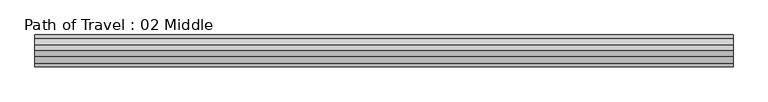
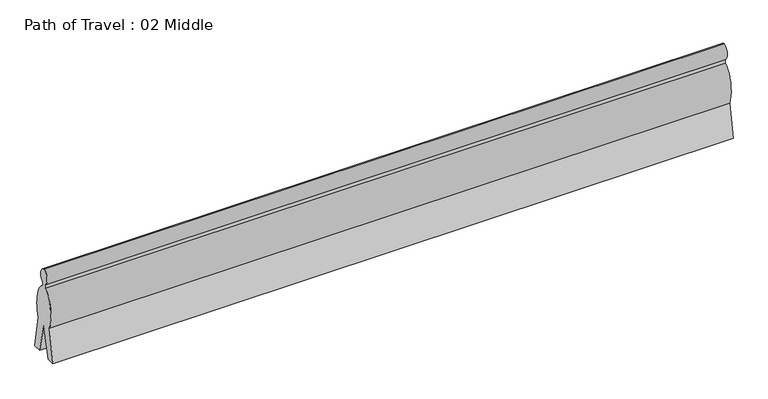
"""IFC4 building model written with IfcOpenShell, lengths in millimetres: proxy geometry, Path of Travel : 02 Middle."""

import ifcopenshell
import ifcopenshell.guid

model = None  # the IFC model being written
_history = None  # IfcOwnerHistory: only IFC2X3 demands one
_inside = {}  # id of a spatial element -> (the spatial element, [elements in it])
_under = {}  # id of a project, library or spatial element -> (it, [spatial elements below it])
_declared = {}  # id of a project -> (the project, [libraries it declares])
_typed = {}  # id of a type object -> (the type object, [elements of that type])
_made_of = {}  # id of a material, layer set ... -> (it, [elements and type objects made of it])


def new_model(schema):
    """Start an empty IFC model of exactly this schema.

    Asked for "IFC4X3", IfcOpenShell would pick the latest addendum, in which some entities
    have other attributes; the version numbers below select the first issue.
    IFC2X3 requires an IfcOwnerHistory on every rooted entity: one is made here for all.
    """
    global model, _history
    if schema == "IFC4X3":
        model = ifcopenshell.file(schema_version=(4, 3, 0, 0))
    else:
        model = ifcopenshell.file(schema=schema)
    _inside.clear()
    _under.clear()
    _declared.clear()
    _typed.clear()
    _made_of.clear()
    _history = None
    if model.schema == "IFC2X3":
        org = make("IfcOrganization", Name="unknown")
        user = make(
            "IfcPersonAndOrganization",
            ThePerson=make("IfcPerson", FamilyName="unknown"),
            TheOrganization=org,
        )
        app = make(
            "IfcApplication",
            ApplicationDeveloper=org,
            Version="unknown",
            ApplicationFullName="unknown",
            ApplicationIdentifier="unknown",
        )
        _history = make(
            "IfcOwnerHistory",
            OwningUser=user,
            OwningApplication=app,
            ChangeAction="ADDED",
            CreationDate=0,
        )
    return model


def make(cls, **values):
    """One entity of the class cls with the attributes given. An attribute that is None is left unset."""
    return model.create_entity(
        cls, **{name: value for name, value in values.items() if value is not None}
    )


def rooted(cls, **values):
    """An entity with a GlobalId (a new one), such as an element, a storey or a relation."""
    return make(cls, GlobalId=ifcopenshell.guid.new(), OwnerHistory=_history, **values)


def si_unit(unit_type, name, prefix=None):
    """IfcSIUnit, for example si_unit("LENGTHUNIT", "METRE", prefix="MILLI")."""
    return make("IfcSIUnit", UnitType=unit_type, Prefix=prefix, Name=name)


def assignment(units):
    """IfcUnitAssignment: the units of a project."""
    return None if units is None else make("IfcUnitAssignment", Units=units)


def point(xyz):
    """IfcCartesianPoint."""
    return None if xyz is None else make("IfcCartesianPoint", Coordinates=xyz)


def direction(xyz):
    """IfcDirection."""
    return None if xyz is None else make("IfcDirection", DirectionRatios=xyz)


def frame(location, z_axis=None, x_axis=None):
    """IfcAxis2Placement3D, a coordinate frame: its origin and axes. An axis left out is left unset."""
    return make(
        "IfcAxis2Placement3D",
        Location=point(location),
        Axis=direction(z_axis),
        RefDirection=direction(x_axis),
    )


def origin():
    """The frame at (0, 0, 0) with its axes left unset."""
    return frame((0.0, 0.0, 0.0))


def place(relative_to, where):
    """IfcLocalPlacement: puts the frame where relative to a parent placement (None: the world)."""
    return make(
        "IfcLocalPlacement", PlacementRelTo=relative_to, RelativePlacement=where
    )


def context(
    kind, dimensions, precision=None, world=None, true_north=None, identifier=None
):
    """IfcGeometricRepresentationContext, for example the 3D "Model" context."""
    return make(
        "IfcGeometricRepresentationContext",
        ContextIdentifier=identifier,
        ContextType=kind,
        CoordinateSpaceDimension=dimensions,
        Precision=precision,
        WorldCoordinateSystem=world,
        TrueNorth=true_north,
    )


def project(units=None, contexts=None):
    """IfcProject with its units and contexts."""
    return rooted(
        "IfcProject",
        Name="project",
        RepresentationContexts=contexts,
        UnitsInContext=assignment(units),
    )


def spatial(cls, under=None, at=None, **own):
    """A site, building, storey or space (cls), placed at a placement, below another one or the project."""
    s = rooted(cls, ObjectPlacement=at, **own)
    if under is not None:
        _under.setdefault(under.id(), (under, []))[1].append(s)
    return s


def ellipse_curve(where, semi_axis1, semi_axis2):
    """IfcEllipse in the frame where."""
    return make(
        "IfcEllipse", Position=where, SemiAxis1=semi_axis1, SemiAxis2=semi_axis2
    )


def trimmed(basis, trim1, trim2, sense, master):
    """IfcTrimmedCurve: the piece of a basis curve between two trims."""
    return make(
        "IfcTrimmedCurve",
        BasisCurve=basis,
        Trim1=trim1,
        Trim2=trim2,
        SenseAgreement=sense,
        MasterRepresentation=master,
    )


def shape(context_of_items, identifier, shape_type, items):
    """IfcShapeRepresentation: the items that make up one representation, for example the "Body"."""
    return make(
        "IfcShapeRepresentation",
        ContextOfItems=context_of_items,
        RepresentationIdentifier=identifier,
        RepresentationType=shape_type,
        Items=items,
    )


def source(mapping_origin, context_of_items, identifier, shape_type, items):
    """IfcRepresentationMap: a shape defined once, which mapped items show again and again."""
    return make(
        "IfcRepresentationMap",
        MappingOrigin=mapping_origin,
        MappedRepresentation=shape(context_of_items, identifier, shape_type, items),
    )


def transform(
    local_origin,
    x_axis=None,
    y_axis=None,
    z_axis=None,
    scale=None,
    scale2=None,
    scale3=None,
    uniform=True,
):
    """IfcCartesianTransformationOperator3D, or its non-uniform kind. x_axis, y_axis, z_axis: its Axis1, 2, 3."""
    if uniform:
        return make(
            "IfcCartesianTransformationOperator3D",
            Axis1=direction(x_axis),
            Axis2=direction(y_axis),
            LocalOrigin=point(local_origin),
            Scale=scale,
            Axis3=direction(z_axis),
        )
    return make(
        "IfcCartesianTransformationOperator3DnonUniform",
        Axis1=direction(x_axis),
        Axis2=direction(y_axis),
        LocalOrigin=point(local_origin),
        Scale=scale,
        Axis3=direction(z_axis),
        Scale2=scale2,
        Scale3=scale3,
    )


def mapped(mapping_source, mapping_target):
    """IfcMappedItem: shows the shape of a source again, moved by a transform."""
    return make(
        "IfcMappedItem", MappingSource=mapping_source, MappingTarget=mapping_target
    )


def made_of(thing, what):
    """Note that an element or type object is made of a material, layer set ...; save() writes the relation."""
    if what is not None:
        _made_of.setdefault(what.id(), (what, []))[1].append(thing)
    return thing


def element(
    cls,
    number,
    at=None,
    inside=None,
    cuts=None,
    type_object=None,
    material=None,
    context=None,
    identifier="Body",
    shape_type=None,
    held_by="IfcProductDefinitionShape",
    body=None,
    shapes=None,
    **own,
):
    """One element of the class cls, such as IfcWall. Its Tag is "e" and its number.

    at: its placement. inside: the storey or other place that contains it. cuts: it is an
    opening in that element (IfcRelVoidsElement). A single representation is given by context,
    identifier, shape_type and body (its items); several are given by shapes. held_by: the class
    of the entity that holds the representations. save() writes the other relations.
    """
    e = rooted(cls, Tag="e%d" % number, ObjectPlacement=at, **own)
    if body is not None:
        shapes = [shape(context, identifier, shape_type, body)]
    if shapes is not None:
        e.Representation = make(held_by, Representations=shapes)
    if inside is not None:
        _inside.setdefault(inside.id(), (inside, []))[1].append(e)
    if cuts is not None:
        rooted(
            "IfcRelVoidsElement", RelatingBuildingElement=cuts, RelatedOpeningElement=e
        )
    if type_object is not None:
        _typed.setdefault(type_object.id(), (type_object, []))[1].append(e)
    return made_of(e, material)


def aggregate(whole, parts):
    """IfcRelAggregates: a whole, such as a stair, and the parts it consists of."""
    return rooted("IfcRelAggregates", RelatingObject=whole, RelatedObjects=parts)


def save(model, path):
    """Write the relations noted so far, then the file.

    IfcRelAggregates (storeys below a building ...), IfcRelContainedInSpatialStructure (elements
    in a storey), IfcRelDefinesByType, IfcRelAssociatesMaterial and IfcRelDeclares: one each for
    every whole, place, type object, material and project.
    """
    for whole, parts in _under.values():
        aggregate(whole, parts)
    for where, things in _inside.values():
        rooted(
            "IfcRelContainedInSpatialStructure",
            RelatedElements=things,
            RelatingStructure=where,
        )
    for kind, things in _typed.values():
        rooted("IfcRelDefinesByType", RelatedObjects=things, RelatingType=kind)
    for what, things in _made_of.values():
        rooted("IfcRelAssociatesMaterial", RelatedObjects=things, RelatingMaterial=what)
    for by, libraries in _declared.values():
        rooted("IfcRelDeclares", RelatingContext=by, RelatedDefinitions=libraries)
    model.write(path)


def plane_surface(at):
    """IfcPlane: the flat surface through the origin of the frame at, square to its z axis."""
    return make("IfcPlane", Position=at)


def extruded_surface(curve, direction_of_extrusion, depth):
    """IfcSurfaceOfLinearExtrusion: the curve pushed along a direction by depth."""
    return make(
        "IfcSurfaceOfLinearExtrusion",
        SweptCurve=make("IfcArbitraryOpenProfileDef", ProfileType="CURVE", Curve=curve),
        ExtrudedDirection=direction(direction_of_extrusion),
        Depth=depth,
    )


def advanced_brep(points, edges, surfaces, faces):
    """IfcAdvancedBrep: a solid bounded by faces that lie on surfaces and meet in shared edges.

    An edge is (start, end): straight between two places in points (the first is 0);
    or (start, end, curve); or (start, end, curve, False) where it runs against its curve.
    A face is (place in surfaces, loops), or (place, loops, False) where it looks against
    its surface's normal. A loop lists edges by number (the first is 1), with a minus sign
    where the edge is run from its end to its start. The first loop is the outer one.
    """
    corners = [point(p) for p in points]
    vertices = [make("IfcVertexPoint", VertexGeometry=c) for c in corners]
    made = []
    for start, end, *more in edges:
        made.append(
            make(
                "IfcEdgeCurve",
                EdgeStart=vertices[start],
                EdgeEnd=vertices[end],
                EdgeGeometry=more[0] if more else make("IfcPolyline", Points=[corners[start], corners[end]]),
                SameSense=more[1] if len(more) > 1 else True,
            )
        )
    hull = []
    for where, loops, *sense in faces:
        bounds = []
        for j, loop in enumerate(loops):
            ring = [make("IfcOrientedEdge", EdgeElement=made[abs(k) - 1], Orientation=k > 0) for k in loop]
            bounds.append(
                make(
                    "IfcFaceOuterBound" if j == 0 else "IfcFaceBound",
                    Bound=make("IfcEdgeLoop", EdgeList=ring),
                    Orientation=True,
                )
            )
        hull.append(make("IfcAdvancedFace", Bounds=bounds, FaceSurface=surfaces[where], SameSense=sense[0] if sense else True))
    return make("IfcAdvancedBrep", Outer=make("IfcClosedShell", CfsFaces=hull))


def path_of_travel_02_middle_d0a210c0(model_context):
    return source(origin(), model_context, "Body", "AdvancedBrep", [
        advanced_brep(
        [(227.5554837, 0.0, 1727.2), (227.5554837, 42.9018657, 1436.6534209), (227.5554837, 42.9018657, 1363.4763406), (227.5554837, 184.1186263, 643.4144547), (227.5554837, 297.5699544, 0.0), (227.5554837, 145.6574193, 0.0), (227.5554837, 0.0, 584.2), (227.5554837, -145.6574193, 0.0), (227.5554837, -297.5699544, 0.0), (227.5554837, -184.1186263, 643.4144547), (227.5554837, -42.9018657, 1363.4763406), (227.5554837, -42.9018657, 1436.6534209), (13204.6046068, 0.0, 1727.2), (13204.6046068, -42.9018657, 1436.6534209), (13204.6046068, -42.9018657, 1363.4763406), (13204.6046068, -184.1186263, 643.4144547), (13204.6046068, -297.5699544, 0.0), (13204.6046068, -145.6574193, 0.0), (13204.6046068, 0.0, 584.2), (13204.6046068, 145.6574193, 0.0), (13204.6046068, 297.5699544, 0.0), (13204.6046068, 184.1186263, 643.4144547), (13204.6046068, 42.9018657, 1363.4763406), (13204.6046068, 42.9018657, 1436.6534209)],
        [
            (0, 1, ellipse_curve(frame((227.5554837, 0.0, 1574.8), z_axis=(-1.0, 0.0, 0.0), x_axis=(0.0, 0.0, 1.0)), 152.4, 101.6)),
            (1, 2),
            (2, 3, ellipse_curve(frame((227.5554837, 0.0, 914.4), z_axis=(-1.0, 0.0, 0.0), x_axis=(0.0, 0.0, -1.0)), 457.2, 228.6)),
            (3, 4),
            (4, 5),
            (5, 6),
            (6, 7),
            (7, 8),
            (8, 9),
            (9, 10, ellipse_curve(frame((227.5554837, 0.0, 914.4), z_axis=(-1.0, 0.0, 0.0), x_axis=(0.0, 0.0, -1.0)), 457.2, 228.6)),
            (10, 11),
            (11, 0, ellipse_curve(frame((227.5554837, 0.0, 1574.8), z_axis=(-1.0, 0.0, 0.0), x_axis=(0.0, 0.0, 1.0)), 152.4, 101.6)),
            (12, 13, ellipse_curve(frame((13204.6046068, 0.0, 1574.8), z_axis=(1.0, 0.0, 0.0), x_axis=(0.0, 0.0, 1.0)), 152.4, 101.6)),
            (13, 14),
            (14, 15, ellipse_curve(frame((13204.6046068, 0.0, 914.4), z_axis=(1.0, 0.0, 0.0), x_axis=(0.0, 0.0, -1.0)), 457.2, 228.6)),
            (15, 16),
            (16, 17),
            (17, 18),
            (18, 19),
            (19, 20),
            (20, 21),
            (21, 22, ellipse_curve(frame((13204.6046068, 0.0, 914.4), z_axis=(1.0, 0.0, 0.0), x_axis=(0.0, 0.0, -1.0)), 457.2, 228.6)),
            (22, 23),
            (23, 12, ellipse_curve(frame((13204.6046068, 0.0, 1574.8), z_axis=(1.0, 0.0, 0.0), x_axis=(0.0, 0.0, 1.0)), 152.4, 101.6)),
            (0, 12),
            (23, 1),
            (22, 2),
            (21, 3),
            (20, 4),
            (19, 5),
            (18, 6),
            (17, 7),
            (16, 8),
            (15, 9),
            (14, 10),
            (13, 11),
        ],
        [
            plane_surface(frame((227.5554837, 0.0, 0.0), z_axis=(-1.0, 0.0, 0.0), x_axis=(0.0, 0.0, 1.0))),
            plane_surface(frame((13204.6046068, 0.0, 0.0), z_axis=(1.0, 0.0, 0.0), x_axis=(0.0, 0.0, 1.0))),
            extruded_surface(trimmed(ellipse_curve(frame((13204.6046068, 0.0, 1574.8), z_axis=(-1.0, 0.0, 0.0), x_axis=(0.0, 0.0, 1.0)), 152.4, 101.6), [point((13204.6046068, 0.0, 1727.2))], [point((13204.6046068, 42.9018657, 1436.6534209))], True, "CARTESIAN"), (-12977.0491231, 0.0, 0.0), 12977.0491231),
            plane_surface(frame((227.5554837, 42.9018657, 1436.6534209), z_axis=(0.0, 1.0, 0.0), x_axis=(1.0, 0.0, 0.0))),
            extruded_surface(trimmed(ellipse_curve(frame((13204.6046068, 0.0, 914.4), z_axis=(-1.0, 0.0, 0.0), x_axis=(0.0, 0.0, -1.0)), 457.2, 228.6), [point((13204.6046068, 42.9018657, 1363.4763406))], [point((13204.6046068, 184.1186263, 643.4144547))], True, "CARTESIAN"), (-12977.0491231, 0.0, 0.0), 12977.0491231),
            plane_surface(frame((227.5554837, 184.1186263, 643.4144547), z_axis=(0.0, 0.9848077530122078, 0.17364817766693205), x_axis=(1.0, 0.0, 0.0))),
            plane_surface(frame((227.5554837, 297.5699544, 0.0), z_axis=(0.0, 0.0, -1.0), x_axis=(1.0, 0.0, 0.0))),
            plane_surface(frame((227.5554837, 145.6574193, 0.0), z_axis=(0.0, -0.9702957262760199, -0.2419218955995739), x_axis=(1.0, 0.0, 0.0))),
            plane_surface(frame((227.5554837, 0.0, 584.2), z_axis=(0.0, 0.9702957262759961, -0.24192189559966923), x_axis=(1.0, 0.0, 0.0))),
            plane_surface(frame((227.5554837, -145.6574193, 0.0), z_axis=(0.0, 0.0, -1.0), x_axis=(1.0, 0.0, 0.0))),
            plane_surface(frame((227.5554837, -297.5699544, 0.0), z_axis=(0.0, -0.984807753012208, 0.17364817766693066), x_axis=(1.0, 0.0, 0.0))),
            extruded_surface(trimmed(ellipse_curve(frame((13204.6046068, 0.0, 914.4), z_axis=(-1.0, 0.0, 0.0), x_axis=(0.0, 0.0, -1.0)), 457.2, 228.6), [point((13204.6046068, -184.1186263, 643.4144547))], [point((13204.6046068, -42.9018657, 1363.4763406))], True, "CARTESIAN"), (-12977.0491231, 0.0, 0.0), 12977.0491231),
            plane_surface(frame((227.5554837, -42.9018657, 1363.4763406), z_axis=(0.0, -1.0, 0.0), x_axis=(1.0, 0.0, 0.0))),
            extruded_surface(trimmed(ellipse_curve(frame((13204.6046068, 0.0, 1574.8), z_axis=(-1.0, 0.0, 0.0), x_axis=(0.0, 0.0, 1.0)), 152.4, 101.6), [point((13204.6046068, -42.9018657, 1436.6534209))], [point((13204.6046068, 0.0, 1727.2))], True, "CARTESIAN"), (-12977.0491231, 0.0, 0.0), 12977.0491231),
        ],
        [
            (0, [[1, 2, 3, 4, 5, 6, 7, 8, 9, 10, 11, 12]]),
            (1, [[13, 14, 15, 16, 17, 18, 19, 20, 21, 22, 23, 24]]),
            (2, [[-1, 25, -24, 26]]),
            (3, [[-2, -26, -23, 27]]),
            (4, [[-3, -27, -22, 28]]),
            (5, [[-4, -28, -21, 29]]),
            (6, [[-5, -29, -20, 30]]),
            (7, [[-6, -30, -19, 31]]),
            (8, [[-7, -31, -18, 32]]),
            (9, [[-8, -32, -17, 33]]),
            (10, [[-9, -33, -16, 34]]),
            (11, [[-10, -34, -15, 35]]),
            (12, [[-11, -35, -14, 36]]),
            (13, [[-12, -36, -13, -25]]),
        ],
    ),
    ])


if __name__ == "__main__":
    model = new_model("IFC4")
    model_context = context("Model", 3, world=origin())
    ifc_project = project(units=[si_unit("LENGTHUNIT", "METRE", prefix="MILLI")], contexts=[model_context])
    site = spatial("IfcSite", under=ifc_project)
    building = spatial("IfcBuilding", under=site)
    placement = place(None, origin())
    path_of_travel_02_middle_shape = path_of_travel_02_middle_d0a210c0(model_context)
    element("IfcBuildingElementProxy", 1, Name="Path of Travel : 02 Middle", ObjectType="Path of Travel : 02 Middle", at=placement, inside=building, context=model_context, shape_type="MappedRepresentation", body=[
        mapped(path_of_travel_02_middle_shape, transform((0.0, 0.0, 0.0), x_axis=(1.0, 0.0, 0.0), y_axis=(0.0, 1.0, 0.0), z_axis=(0.0, 0.0, 1.0))),
    ])
    save(model, "model.ifc")

# Revit data of these elements
# Type "Path of Travel : 02 Middle"
#   Path of Egress [instance default] = 4' - 0"
#   built-in parameter 1001306 [instance default] = 4 (stored number, unit not read)
#   Dot at Start = no
#   Arrow in Middle = yes
#   Arrow at End = no
#   Egress Path = none
# Element 1 (IfcBuildingElementProxy, "Path of Travel : 02 Middle")
#   Path of Egress = 42' - 6.90745"
#   built-in parameter 1001306 = 42.5756 (stored number, unit not read)
#   Materials on its faces: "Egress Path Solid"
# Materials
#   "Egress Path Solid": class "Unassigned", colour RGB 255 128 64, transparency 0.75, Comments = "Rendering appearance not upgraded "
